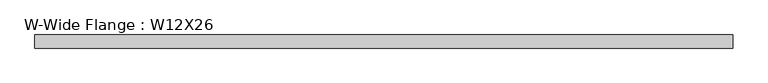
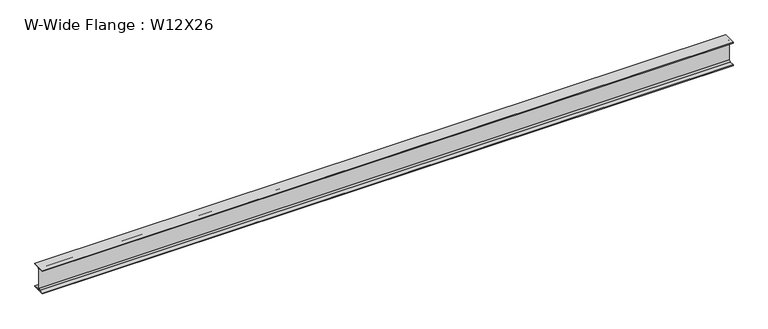
"""IFC4 building model written with IfcOpenShell, lengths in millimetres: beam geometry, W-Wide Flange : W12X26."""

from ifc_helpers import new_model, si_unit, point, frame, frame_2d, origin, place, context, project, spatial, polyline, circle_curve, trimmed, segment, composite_curve, outline, extrude, source, transform, mapped, element, save


def w_wide_flange_w12x26_5caf9ca6(model_context):
    return source(origin(), model_context, "Body", "SweptSolid", [
        extrude(outline(composite_curve([segment(polyline([(82.4011719, -145.5539063), (82.4011719, -155.178125), (-82.4011719, -155.178125), (-82.4011719, -145.5539063), (-20.2902344, -145.5539063)]), True, "CONTINUOUS"), segment(trimmed(circle_curve(frame_2d((-20.2902344, -128.190625)), 17.3632812), [point((-20.2902344, -145.5539063))], [point((-2.9269531, -128.190625))], True, "CARTESIAN"), True, "CONTINUOUS"), segment(polyline([(-2.9269531, -128.190625), (-2.9269531, 128.190625)]), True, "CONTINUOUS"), segment(trimmed(circle_curve(frame_2d((-20.2902344, 128.190625)), 17.3632812), [point((-2.9269531, 128.190625))], [point((-20.2902344, 145.5539062))], True, "CARTESIAN"), True, "CONTINUOUS"), segment(polyline([(-20.2902344, 145.5539062), (-82.4011719, 145.5539062), (-82.4011719, 155.178125), (82.4011719, 155.178125), (82.4011719, 145.5539062), (20.2902344, 145.5539062)]), True, "CONTINUOUS"), segment(trimmed(circle_curve(frame_2d((20.2902344, 128.190625)), 17.3632812), [point((20.2902344, 145.5539062))], [point((2.9269531, 128.190625))], True, "CARTESIAN"), True, "CONTINUOUS"), segment(polyline([(2.9269531, 128.190625), (2.9269531, -128.190625)]), True, "CONTINUOUS"), segment(trimmed(circle_curve(frame_2d((20.2902344, -128.190625)), 17.3632812), [point((2.9269531, -128.190625))], [point((20.2902344, -145.5539063))], True, "CARTESIAN"), True, "CONTINUOUS"), segment(polyline([(20.2902344, -145.5539063), (82.4011719, -145.5539063)]), True, "CONTINUOUS")], self_intersect=False)), frame((-4279.8812527, 0.0, 0.0), z_axis=(1.0, 0.0, 0.0), x_axis=(0.0, 1.0, 0.0)), (0.0, 0.0, 1.0), 8737.2648492),
    ])


if __name__ == "__main__":
    model = new_model("IFC4")
    model_context = context("Model", 3, world=origin())
    ifc_project = project(units=[si_unit("LENGTHUNIT", "METRE", prefix="MILLI")], contexts=[model_context])
    site = spatial("IfcSite", under=ifc_project)
    building = spatial("IfcBuilding", under=site)
    placement = place(None, origin())
    w_wide_flange_w12x26_shape = w_wide_flange_w12x26_5caf9ca6(model_context)
    element("IfcBeam", 1, ObjectType="W-Wide Flange : W12X26", at=placement, inside=building, context=model_context, shape_type="MappedRepresentation", body=[
        mapped(w_wide_flange_w12x26_shape, transform((0.0, 0.0, 0.0), x_axis=(1.0, 0.0, 0.0), y_axis=(0.0, 1.0, 0.0), z_axis=(0.0, 0.0, 1.0))),
    ])
    save(model, "model.ifc")

# Revit data of these elements
# Type "W-Wide Flange : W12X26"
#   Assembly Code = "B10"
#   W = 26
#   Length [instance default] = 5' - 0"
#   bf = 0' - 6 125/256"
#   d = 1' - 0 7/32"
#   k = 0' - 1 1/16"
#   k2 = 0' - 0 175/256"
#   tf = 0' - 0 97/256"
#   tw = 0' - 0 59/256"
#   A = 0.053125 SF
#   Structural Material [instance default] = none
# Element 1 (IfcBeam, "W-Wide Flange : W12X26")
#   Structural Material = Dark metal
#   Materials on its faces: "Dark metal"
# Materials
#   "Dark metal": class "Generic", colour RGB 44 29 29, transparency 0, Cost = 0
